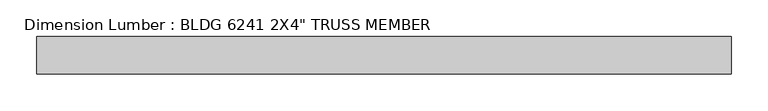
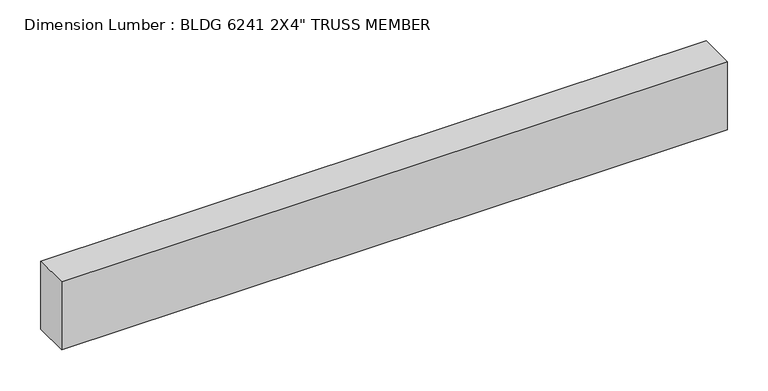
"""IFC4 building model written with IfcOpenShell, lengths in millimetres: beam geometry."""

from ifc_helpers import new_model, si_unit, frame, origin, place, context, project, spatial, polyline, outline, extrude, source, transform, mapped, element, save


def beam_c7262e2a(model_context):
    return source(origin(), model_context, "Body", "SweptSolid", [
        extrude(outline(polyline([(450.6043361, 25.4), (450.6043361, -25.4), (-488.5308943, -25.4), (-488.5308943, 25.4), (450.6043361, 25.4)])), frame((0.0, 0.0, -50.8), z_axis=(0.0, 0.0, 1.0), x_axis=(1.0, 0.0, 0.0)), (0.0, 0.0, 1.0), 101.6),
    ])


if __name__ == "__main__":
    model = new_model("IFC4")
    model_context = context("Model", 3, world=origin())
    ifc_project = project(units=[si_unit("LENGTHUNIT", "METRE", prefix="MILLI")], contexts=[model_context])
    site = spatial("IfcSite", under=ifc_project)
    building = spatial("IfcBuilding", under=site)
    placement = place(None, origin())
    beam_shape = beam_c7262e2a(model_context)
    element("IfcBeam", 1, ObjectType="Dimension Lumber : BLDG 6241 2X4\" TRUSS MEMBER", at=placement, inside=building, context=model_context, shape_type="MappedRepresentation", body=[
        mapped(beam_shape, transform((0.0, 0.0, 0.0), x_axis=(1.0, 0.0, 0.0), y_axis=(0.0, 1.0, 0.0), z_axis=(0.0, 0.0, 1.0))),
    ])
    save(model, "model.ifc")

# Revit data of these elements
# Type "Dimension Lumber : BLDG 6241 2X4\" TRUSS MEMBER"
#   Assembly Code = "B10"
#   A = 0.273472 SF
#   Length [instance default] = 5' - 0"
#   b = 0' - 2"
#   d = 0' - 4"
#   Structural Material [instance default] = Softwood, Lumber
# Element 1 (IfcBeam, "Dimension Lumber : BLDG 6241 2X4\" TRUSS MEMBER")
#   Materials on its faces: "Softwood, Lumber"
# Materials
#   "Softwood, Lumber": class "Wood", colour RGB 223 192 134, transparency 0, Description = "Pinus Echinata", Cost = 0
